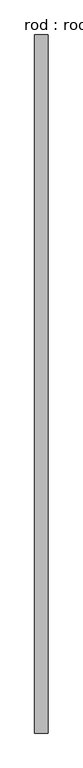
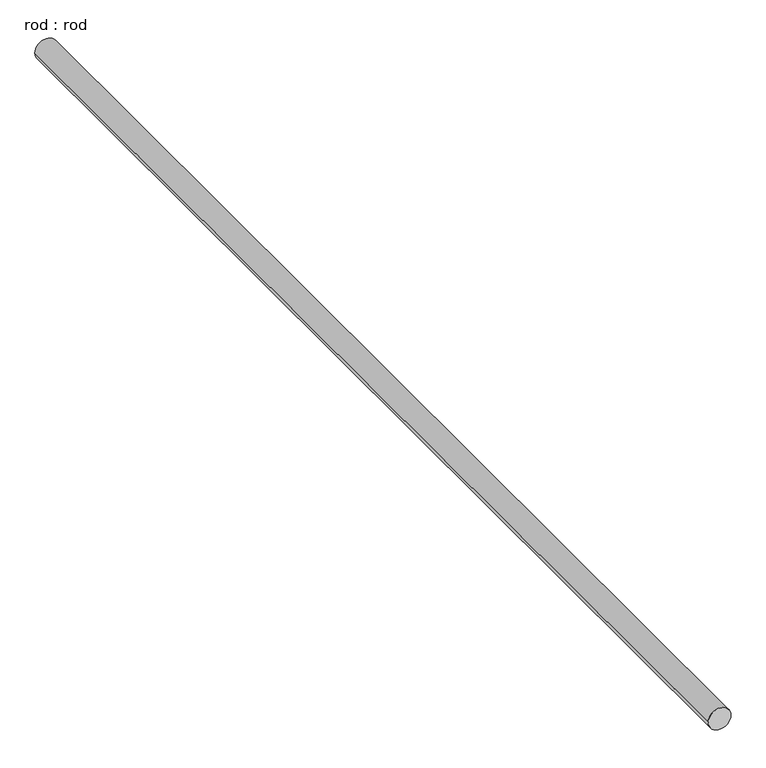
"""IFC4 building model written with IfcOpenShell, lengths in millimetres: proxy geometry, rod : rod."""

import ifcopenshell
import ifcopenshell.guid

model = None  # the IFC model being written
_history = None  # IfcOwnerHistory: only IFC2X3 demands one
_inside = {}  # id of a spatial element -> (the spatial element, [elements in it])
_under = {}  # id of a project, library or spatial element -> (it, [spatial elements below it])
_declared = {}  # id of a project -> (the project, [libraries it declares])
_typed = {}  # id of a type object -> (the type object, [elements of that type])
_made_of = {}  # id of a material, layer set ... -> (it, [elements and type objects made of it])


def new_model(schema):
    """Start an empty IFC model of exactly this schema.

    Asked for "IFC4X3", IfcOpenShell would pick the latest addendum, in which some entities
    have other attributes; the version numbers below select the first issue.
    IFC2X3 requires an IfcOwnerHistory on every rooted entity: one is made here for all.
    """
    global model, _history
    if schema == "IFC4X3":
        model = ifcopenshell.file(schema_version=(4, 3, 0, 0))
    else:
        model = ifcopenshell.file(schema=schema)
    _inside.clear()
    _under.clear()
    _declared.clear()
    _typed.clear()
    _made_of.clear()
    _history = None
    if model.schema == "IFC2X3":
        org = make("IfcOrganization", Name="unknown")
        user = make(
            "IfcPersonAndOrganization",
            ThePerson=make("IfcPerson", FamilyName="unknown"),
            TheOrganization=org,
        )
        app = make(
            "IfcApplication",
            ApplicationDeveloper=org,
            Version="unknown",
            ApplicationFullName="unknown",
            ApplicationIdentifier="unknown",
        )
        _history = make(
            "IfcOwnerHistory",
            OwningUser=user,
            OwningApplication=app,
            ChangeAction="ADDED",
            CreationDate=0,
        )
    return model


def make(cls, **values):
    """One entity of the class cls with the attributes given. An attribute that is None is left unset."""
    return model.create_entity(
        cls, **{name: value for name, value in values.items() if value is not None}
    )


def rooted(cls, **values):
    """An entity with a GlobalId (a new one), such as an element, a storey or a relation."""
    return make(cls, GlobalId=ifcopenshell.guid.new(), OwnerHistory=_history, **values)


def si_unit(unit_type, name, prefix=None):
    """IfcSIUnit, for example si_unit("LENGTHUNIT", "METRE", prefix="MILLI")."""
    return make("IfcSIUnit", UnitType=unit_type, Prefix=prefix, Name=name)


def assignment(units):
    """IfcUnitAssignment: the units of a project."""
    return None if units is None else make("IfcUnitAssignment", Units=units)


def point(xyz):
    """IfcCartesianPoint."""
    return None if xyz is None else make("IfcCartesianPoint", Coordinates=xyz)


def direction(xyz):
    """IfcDirection."""
    return None if xyz is None else make("IfcDirection", DirectionRatios=xyz)


def frame(location, z_axis=None, x_axis=None):
    """IfcAxis2Placement3D, a coordinate frame: its origin and axes. An axis left out is left unset."""
    return make(
        "IfcAxis2Placement3D",
        Location=point(location),
        Axis=direction(z_axis),
        RefDirection=direction(x_axis),
    )


def frame_2d(location, x_axis=None):
    """IfcAxis2Placement2D, a coordinate frame in the plane: its origin and x axis."""
    return make(
        "IfcAxis2Placement2D", Location=point(location), RefDirection=direction(x_axis)
    )


def origin():
    """The frame at (0, 0, 0) with its axes left unset."""
    return frame((0.0, 0.0, 0.0))


def place(relative_to, where):
    """IfcLocalPlacement: puts the frame where relative to a parent placement (None: the world)."""
    return make(
        "IfcLocalPlacement", PlacementRelTo=relative_to, RelativePlacement=where
    )


def context(
    kind, dimensions, precision=None, world=None, true_north=None, identifier=None
):
    """IfcGeometricRepresentationContext, for example the 3D "Model" context."""
    return make(
        "IfcGeometricRepresentationContext",
        ContextIdentifier=identifier,
        ContextType=kind,
        CoordinateSpaceDimension=dimensions,
        Precision=precision,
        WorldCoordinateSystem=world,
        TrueNorth=true_north,
    )


def project(units=None, contexts=None):
    """IfcProject with its units and contexts."""
    return rooted(
        "IfcProject",
        Name="project",
        RepresentationContexts=contexts,
        UnitsInContext=assignment(units),
    )


def spatial(cls, under=None, at=None, **own):
    """A site, building, storey or space (cls), placed at a placement, below another one or the project."""
    s = rooted(cls, ObjectPlacement=at, **own)
    if under is not None:
        _under.setdefault(under.id(), (under, []))[1].append(s)
    return s


def circle_curve(where, radius):
    """IfcCircle in the frame where."""
    return make("IfcCircle", Position=where, Radius=radius)


def trimmed(basis, trim1, trim2, sense, master):
    """IfcTrimmedCurve: the piece of a basis curve between two trims."""
    return make(
        "IfcTrimmedCurve",
        BasisCurve=basis,
        Trim1=trim1,
        Trim2=trim2,
        SenseAgreement=sense,
        MasterRepresentation=master,
    )


def segment(curve, same_sense, transition):
    """IfcCompositeCurveSegment."""
    return make(
        "IfcCompositeCurveSegment",
        Transition=transition,
        SameSense=same_sense,
        ParentCurve=curve,
    )


def composite_curve(segments, self_intersect=None):
    """IfcCompositeCurve: segments joined end to end."""
    return make("IfcCompositeCurve", Segments=segments, SelfIntersect=self_intersect)


def outline(outer, holes=None, kind="AREA"):
    """IfcArbitraryClosedProfileDef: a profile drawn as a closed curve; with holes, ...WithVoids."""
    if holes is None:
        return make("IfcArbitraryClosedProfileDef", ProfileType=kind, OuterCurve=outer)
    return make(
        "IfcArbitraryProfileDefWithVoids",
        ProfileType=kind,
        OuterCurve=outer,
        InnerCurves=holes,
    )


def extrude(swept, where, along, depth):
    """IfcExtrudedAreaSolid: the profile swept, set in the frame where, extruded along a direction by depth."""
    return make(
        "IfcExtrudedAreaSolid",
        SweptArea=swept,
        Position=where,
        ExtrudedDirection=direction(along),
        Depth=depth,
    )


def shape(context_of_items, identifier, shape_type, items):
    """IfcShapeRepresentation: the items that make up one representation, for example the "Body"."""
    return make(
        "IfcShapeRepresentation",
        ContextOfItems=context_of_items,
        RepresentationIdentifier=identifier,
        RepresentationType=shape_type,
        Items=items,
    )


def source(mapping_origin, context_of_items, identifier, shape_type, items):
    """IfcRepresentationMap: a shape defined once, which mapped items show again and again."""
    return make(
        "IfcRepresentationMap",
        MappingOrigin=mapping_origin,
        MappedRepresentation=shape(context_of_items, identifier, shape_type, items),
    )


def transform(
    local_origin,
    x_axis=None,
    y_axis=None,
    z_axis=None,
    scale=None,
    scale2=None,
    scale3=None,
    uniform=True,
):
    """IfcCartesianTransformationOperator3D, or its non-uniform kind. x_axis, y_axis, z_axis: its Axis1, 2, 3."""
    if uniform:
        return make(
            "IfcCartesianTransformationOperator3D",
            Axis1=direction(x_axis),
            Axis2=direction(y_axis),
            LocalOrigin=point(local_origin),
            Scale=scale,
            Axis3=direction(z_axis),
        )
    return make(
        "IfcCartesianTransformationOperator3DnonUniform",
        Axis1=direction(x_axis),
        Axis2=direction(y_axis),
        LocalOrigin=point(local_origin),
        Scale=scale,
        Axis3=direction(z_axis),
        Scale2=scale2,
        Scale3=scale3,
    )


def mapped(mapping_source, mapping_target):
    """IfcMappedItem: shows the shape of a source again, moved by a transform."""
    return make(
        "IfcMappedItem", MappingSource=mapping_source, MappingTarget=mapping_target
    )


def made_of(thing, what):
    """Note that an element or type object is made of a material, layer set ...; save() writes the relation."""
    if what is not None:
        _made_of.setdefault(what.id(), (what, []))[1].append(thing)
    return thing


def element(
    cls,
    number,
    at=None,
    inside=None,
    cuts=None,
    type_object=None,
    material=None,
    context=None,
    identifier="Body",
    shape_type=None,
    held_by="IfcProductDefinitionShape",
    body=None,
    shapes=None,
    **own,
):
    """One element of the class cls, such as IfcWall. Its Tag is "e" and its number.

    at: its placement. inside: the storey or other place that contains it. cuts: it is an
    opening in that element (IfcRelVoidsElement). A single representation is given by context,
    identifier, shape_type and body (its items); several are given by shapes. held_by: the class
    of the entity that holds the representations. save() writes the other relations.
    """
    e = rooted(cls, Tag="e%d" % number, ObjectPlacement=at, **own)
    if body is not None:
        shapes = [shape(context, identifier, shape_type, body)]
    if shapes is not None:
        e.Representation = make(held_by, Representations=shapes)
    if inside is not None:
        _inside.setdefault(inside.id(), (inside, []))[1].append(e)
    if cuts is not None:
        rooted(
            "IfcRelVoidsElement", RelatingBuildingElement=cuts, RelatedOpeningElement=e
        )
    if type_object is not None:
        _typed.setdefault(type_object.id(), (type_object, []))[1].append(e)
    return made_of(e, material)


def aggregate(whole, parts):
    """IfcRelAggregates: a whole, such as a stair, and the parts it consists of."""
    return rooted("IfcRelAggregates", RelatingObject=whole, RelatedObjects=parts)


def save(model, path):
    """Write the relations noted so far, then the file.

    IfcRelAggregates (storeys below a building ...), IfcRelContainedInSpatialStructure (elements
    in a storey), IfcRelDefinesByType, IfcRelAssociatesMaterial and IfcRelDeclares: one each for
    every whole, place, type object, material and project.
    """
    for whole, parts in _under.values():
        aggregate(whole, parts)
    for where, things in _inside.values():
        rooted(
            "IfcRelContainedInSpatialStructure",
            RelatedElements=things,
            RelatingStructure=where,
        )
    for kind, things in _typed.values():
        rooted("IfcRelDefinesByType", RelatedObjects=things, RelatingType=kind)
    for what, things in _made_of.values():
        rooted("IfcRelAssociatesMaterial", RelatedObjects=things, RelatingMaterial=what)
    for by, libraries in _declared.values():
        rooted("IfcRelDeclares", RelatingContext=by, RelatedDefinitions=libraries)
    model.write(path)


def rod_rod_727f5926(model_context):
    return source(origin(), model_context, "Body", "SweptSolid", [
        extrude(outline(composite_curve([segment(trimmed(circle_curve(frame_2d((0.0108462, 0.0)), 200.0), [point((0.0108462, 200.0))], [point((0.0108462, -200.0))], False, "CARTESIAN"), True, "CONTINUOUS"), segment(trimmed(circle_curve(frame_2d((0.0108462, 0.0)), 200.0), [point((0.0108462, -200.0))], [point((0.0108462, 200.0))], False, "CARTESIAN"), True, "CONTINUOUS")], self_intersect=False)), frame((0.0, -6261.1743323, 0.0), z_axis=(0.0, 1.0, 0.0), x_axis=(0.0, 0.0, 1.0)), (0.0, 0.0, 1.0), 20707.8058954),
    ])


if __name__ == "__main__":
    model = new_model("IFC4")
    model_context = context("Model", 3, world=origin())
    ifc_project = project(units=[si_unit("LENGTHUNIT", "METRE", prefix="MILLI")], contexts=[model_context])
    site = spatial("IfcSite", under=ifc_project)
    building = spatial("IfcBuilding", under=site)
    placement = place(None, origin())
    rod_rod_shape = rod_rod_727f5926(model_context)
    element("IfcBuildingElementProxy", 1, Name="rod : rod", ObjectType="rod : rod", at=placement, inside=building, context=model_context, shape_type="MappedRepresentation", body=[
        mapped(rod_rod_shape, transform((0.0, 0.0, 0.0), x_axis=(1.0, 0.0, 0.0), y_axis=(0.0, 1.0, 0.0), z_axis=(0.0, 0.0, 1.0))),
    ])
    save(model, "model.ifc")

# Revit data of these elements
# Type "rod : rod"
#   Default Elevation = 0
